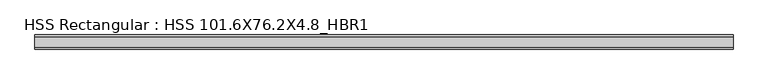
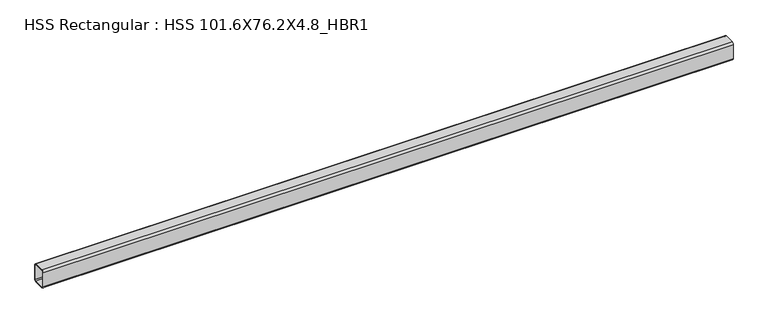
"""IFC4 building model written with IfcOpenShell, lengths in millimetres: beam geometry, HSS Rectangular : HSS 101.6X76.2X4.8_HBR1."""

from ifc_helpers import new_model, si_unit, point, frame, frame_2d, origin, place, context, project, spatial, polyline, circle_curve, trimmed, segment, composite_curve, outline, extrude, source, transform, mapped, element, save


def hss_rectangular_hss_101_6x76_2x4_8_hbr1_df5ea1dc(model_context):
    return source(origin(), model_context, "Body", "SweptSolid", [
        extrude(outline(composite_curve([segment(polyline([(38.1, 41.275), (38.1, -41.275)]), True, "CONTINUOUS"), segment(trimmed(circle_curve(frame_2d((28.575, -41.275)), 9.525), [point((38.1, -41.275))], [point((28.575, -50.8))], False, "CARTESIAN"), True, "CONTINUOUS"), segment(polyline([(28.575, -50.8), (-28.575, -50.8)]), True, "CONTINUOUS"), segment(trimmed(circle_curve(frame_2d((-28.575, -41.275)), 9.525), [point((-28.575, -50.8))], [point((-38.1, -41.275))], False, "CARTESIAN"), True, "CONTINUOUS"), segment(polyline([(-38.1, -41.275), (-38.1, 41.275)]), True, "CONTINUOUS"), segment(trimmed(circle_curve(frame_2d((-28.575, 41.275)), 9.525), [point((-38.1, 41.275))], [point((-28.575, 50.8))], False, "CARTESIAN"), True, "CONTINUOUS"), segment(polyline([(-28.575, 50.8), (28.575, 50.8)]), True, "CONTINUOUS"), segment(trimmed(circle_curve(frame_2d((28.575, 41.275)), 9.525), [point((28.575, 50.8))], [point((38.1, 41.275))], False, "CARTESIAN"), True, "CONTINUOUS")], self_intersect=False), holes=[composite_curve([segment(trimmed(circle_curve(frame_2d((-28.575, 41.275)), 4.7625), [point((-28.575, 46.0375))], [point((-33.3375, 41.275))], True, "CARTESIAN"), True, "CONTINUOUS"), segment(polyline([(-33.3375, 41.275), (-33.3375, -41.275)]), True, "CONTINUOUS"), segment(trimmed(circle_curve(frame_2d((-28.575, -41.275)), 4.7625), [point((-33.3375, -41.275))], [point((-28.575, -46.0375))], True, "CARTESIAN"), True, "CONTINUOUS"), segment(polyline([(-28.575, -46.0375), (28.575, -46.0375)]), True, "CONTINUOUS"), segment(trimmed(circle_curve(frame_2d((28.575, -41.275)), 4.7625), [point((28.575, -46.0375))], [point((33.3375, -41.275))], True, "CARTESIAN"), True, "CONTINUOUS"), segment(polyline([(33.3375, -41.275), (33.3375, 41.275)]), True, "CONTINUOUS"), segment(trimmed(circle_curve(frame_2d((28.575, 41.275)), 4.7625), [point((33.3375, 41.275))], [point((28.575, 46.0375))], True, "CARTESIAN"), True, "CONTINUOUS"), segment(polyline([(28.575, 46.0375), (-28.575, 46.0375)]), True, "CONTINUOUS")], self_intersect=False)]), frame((-1859.9709573, 0.0, 0.0), z_axis=(1.0, 0.0, 0.0), x_axis=(0.0, 1.0, 0.0)), (0.0, 0.0, 1.0), 3761.6288172),
    ])


if __name__ == "__main__":
    model = new_model("IFC4")
    model_context = context("Model", 3, world=origin())
    ifc_project = project(units=[si_unit("LENGTHUNIT", "METRE", prefix="MILLI")], contexts=[model_context])
    site = spatial("IfcSite", under=ifc_project)
    building = spatial("IfcBuilding", under=site)
    placement = place(None, origin())
    hss_rectangular_hss_101_6x76_2x4_8_hbr1_shape = hss_rectangular_hss_101_6x76_2x4_8_hbr1_df5ea1dc(model_context)
    element("IfcBeam", 1, ObjectType="HSS Rectangular : HSS 101.6X76.2X4.8_HBR1", at=placement, inside=building, context=model_context, shape_type="MappedRepresentation", body=[
        mapped(hss_rectangular_hss_101_6x76_2x4_8_hbr1_shape, transform((0.0, 0.0, 0.0), x_axis=(1.0, 0.0, 0.0), y_axis=(0.0, 1.0, 0.0), z_axis=(0.0, 0.0, 1.0))),
    ])
    save(model, "model.ifc")

# Revit data of these elements
# Type "HSS Rectangular : HSS 101.6X76.2X4.8_HBR1"
#   Section Name Key = "HSS 4X3X3/16"
#   Assembly Code = "B10"
#   Width = 7.62 cm
#   Wall Nominal Thickness = 0.4763 cm
#   Wall Design Thickness = 0.442 cm
#   Torsional Moment of Inertia = 260.561 cm⁴
#   Torsional Modulus = 61.2876 cm³
#   Section Area = 14.4516 cm²
#   Plastic Modulus weak axis = 40.3122 cm³
#   Plastic Modulus strong axis = 49.1612 cm³
#   Perimeter = 0.881482 m²/m
#   Outer Fillet = 0.9525 cm
#   Nominal Weight = 12.1285 kgf/m
#   Moment of Inertia weak axis = 131.529 cm⁴
#   Moment of Inertia strong axis = 205.202 cm⁴
#   Inner Fillet = 0.4763 cm
#   Height = 10.16 cm
#   Elastic Modulus weak axis = 34.4128 cm³
#   Elastic Modulus strong axis = 40.476 cm³
#   Centroid Vertical = 5.08 cm
#   Centroid Horizontal = 3.81 cm
#   Length [instance default] = 1524 mm
#   Structural Material [instance default] = Steel ASTM A500, Grade B, Rectangular and Square
#   Principal Axes Angle = 0
# Element 1 (IfcBeam, "HSS Rectangular : HSS 101.6X76.2X4.8_HBR1")
#   Structural Material = Steel ASTM A992
#   Materials on its faces: "Steel ASTM A992"
# Materials
#   "Steel ASTM A500, Grade B, Rectangular and Square": class "Metal", colour RGB 199 199 199, transparency 0, Description = "Carbon steel", Cost = 0
#   "Steel ASTM A992": class "Metal", colour RGB 199 199 199, transparency 0, Description = "Structural steel 50ksi", Cost = 0
